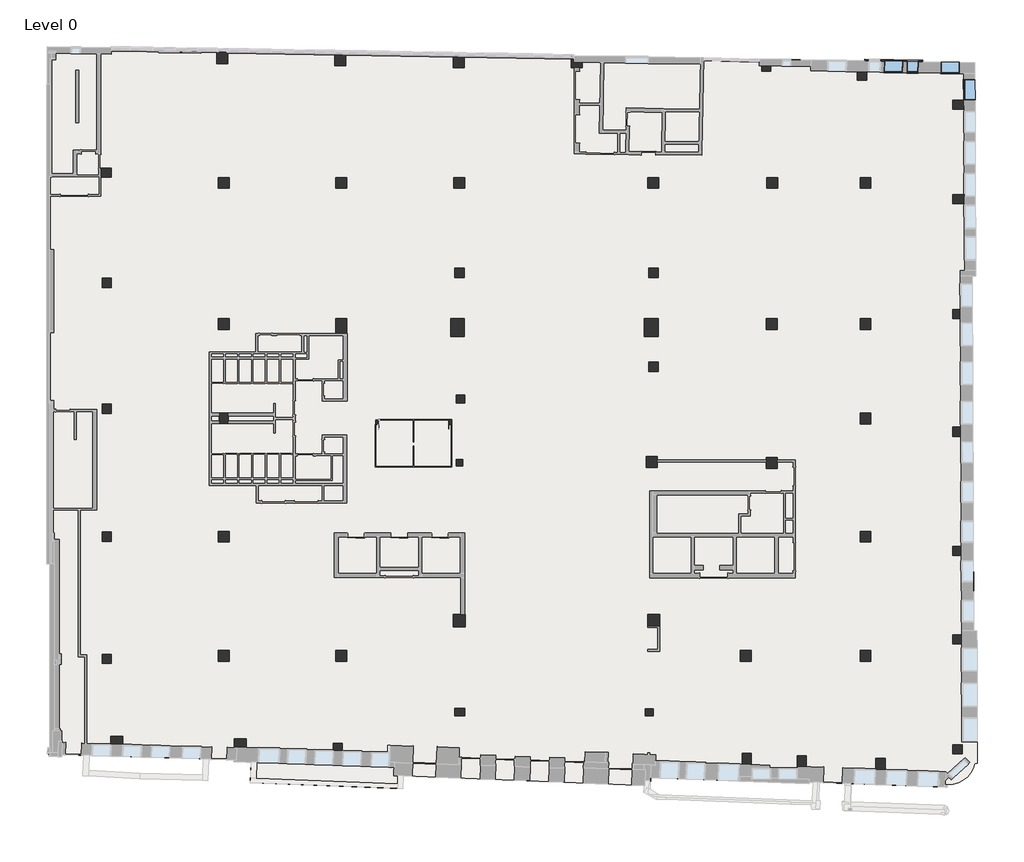
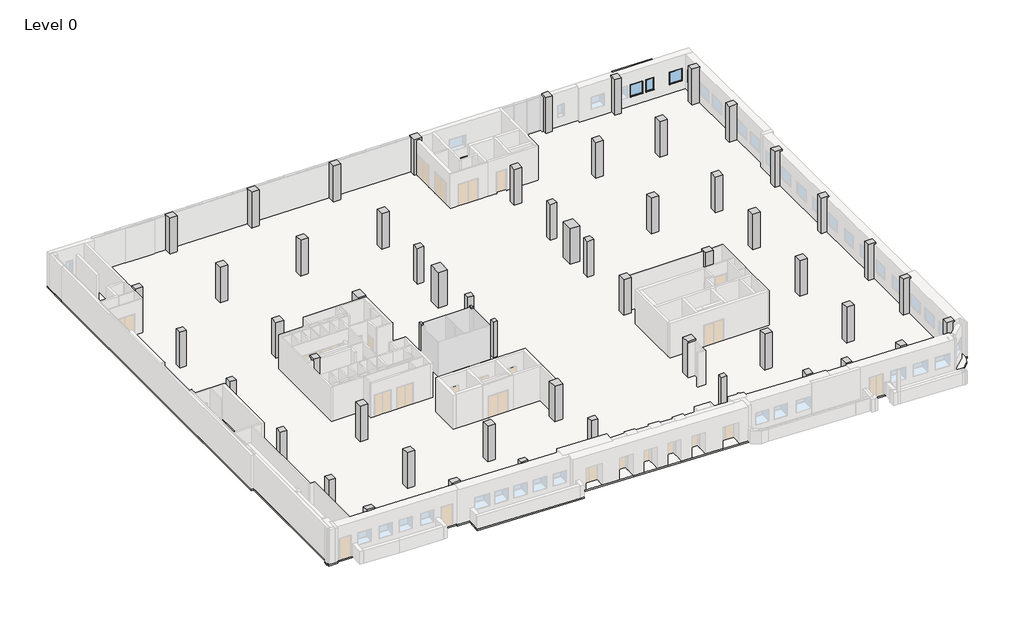
# One storey, part 9 of 9: 57 columns, 4 windows, 1 slab, 1 wall.
# Revit data of these elements (continued)
# Type "WWm-ConcreteRectangular-Instance : Generic" (continued)
#   Material = WW-EC-CR-CastInPlace
#   Assembly Code = ""
# Type "WWm-Existing-Slab-150mm"
#   Layers, outside or top first: 150 mm "WW-EC-CR-CastInPlace" (function 1)
# Type "WWm-Existing-ExtPartition-110mm"
#   Keynote = ""
#   Type IfcGUID = ""
#   Type Comments = ""
#   Description = ""
#   Type Mark = ""
#   Fire Rating = ""
#   Layers, outside or top first: 110 mm "WW-EC-RGB-White" (function 1)
# Type "Window-Instance : 1200x1200"
#   Type Mark = "11"
#   Construction Type Id = "GSP4R"
#   Assembly Code = "B2020100"
#   Analytic Construction = "1/8 in Pilkington single glazing"
#   Visual Light Transmittance = 0.9
#   Thermal Resistance (R) = 0.149095 (m²·K)/W
#   Solar Heat Gain Coefficient = 0.86
#   Heat Transfer Coefficient (U) = 6.70716 W/(m²·K)
#   Height [instance default] = 1200 mm
#   Default Sill Height = 900 mm
#   Width [instance default] = 600 mm
#   Window Inset = 20 mm
#   Glass Pane Material = none
#   Sash Material = none
#   Wall Closure = (empty or 0)
# Type "Window-Instance : 600x1200"
#   Type Mark = "7"
#   Construction Type Id = "GSP4R"
#   Assembly Code = "B2020100"
#   Analytic Construction = "1/8 in Pilkington single glazing"
#   Visual Light Transmittance = 0.9
#   Thermal Resistance (R) = 0.149095 (m²·K)/W
#   Solar Heat Gain Coefficient = 0.86
#   Heat Transfer Coefficient (U) = 6.70716 W/(m²·K)
#   Height [instance default] = 1200 mm
#   Default Sill Height = 900 mm
#   Width [instance default] = 600 mm
#   Window Inset = 20 mm
#   Glass Pane Material = WW-EC-GL-Storefront
#   Sash Material = WW-EC-RGB-White
#   Wall Closure = (empty or 0)
# Element 1 (IfcColumn, "WWm-ConcreteRectangular-Instance : Generic")
#   Width = 696 mm
#   Depth = 714.449 mm
#   Phase Created = Existing
#   Materials on its faces: "WW-EC-CR-CastInPlace", "WW-EC-RGB-White"
# Elements 2, 3, 4 (IfcColumn, "WWm-ConcreteRectangular-Instance : Generic")
#   Width = 696 mm
#   Depth = 692 mm
#   Phase Created = Existing
#   Materials on its faces: "WW-EC-CR-CastInPlace", "WW-EC-RGB-White"
# Elements 5, 6, 12, 19, 20, 21, 22, 23, 25, 26, 27, 29, 30, 31, 32, 33, 40, 57 (IfcColumn, "WWm-ConcreteRectangular-Instance : Generic")
#   Width = 696 mm
#   Depth = 692 mm
#   Phase Created = Existing
#   Materials on its faces: "WW-EC-CR-CastInPlace"
# Elements 7, 50, 51, 52 (IfcColumn, "WWm-ConcreteRectangular-Instance : Generic")
#   Width = 696 mm
#   Depth = 592 mm
#   Phase Created = Existing
#   Materials on its faces: "WW-EC-CR-CastInPlace", "WW-EC-RGB-White"
# Elements 8, 9, 11, 13, 34, 35 (IfcColumn, "WWm-ConcreteRectangular-Instance : Generic")
#   Width = 592 mm
#   Depth = 592 mm
#   Phase Created = Existing
#   Materials on its faces: "WW-EC-CR-CastInPlace"
# Element 10 (IfcColumn, "WWm-ConcreteRectangular-Instance : Generic")
#   Width = 600 mm
#   Depth = 669 mm
#   Phase Created = Existing
#   Materials on its faces: "WW-EC-CR-CastInPlace"
# Element 14 (IfcColumn, "WWm-ConcreteRectangular-Instance : Generic")
#   Width = 750 mm
#   Depth = 521.22 mm
#   Phase Created = Existing
#   Materials on its faces: "WW-EC-CR-CastInPlace", "WW-EC-RGB-White"
# Element 15 (IfcColumn, "WWm-ConcreteRectangular-Instance : Generic")
#   Width = 750 mm
#   Depth = 548.855 mm
#   Phase Created = Existing
#   Materials on its faces: "WW-EC-CR-CastInPlace", "WW-EC-RGB-White"
# Element 16 (IfcColumn, "WWm-ConcreteRectangular-Instance : Generic")
#   Width = 589.75 mm
#   Depth = 455.168 mm
#   Phase Created = Existing
#   Materials on its faces: "WW-EC-CR-CastInPlace", "WW-EC-RGB-White"
# Element 17 (IfcColumn, "WWm-ConcreteRectangular-Instance : Generic")
#   Width = 625.153 mm
#   Depth = 492.025 mm
#   Phase Created = Existing
#   Materials on its faces: "WW-EC-CR-CastInPlace"
# Element 18 (IfcColumn, "WWm-ConcreteRectangular-Instance : Generic")
#   Width = 498.218 mm
#   Depth = 470.145 mm
#   Phase Created = Existing
#   Materials on its faces: "WW-EC-CR-CastInPlace"
# Element 24 (IfcColumn, "WWm-ConcreteRectangular-Instance : Generic")
#   Width = 751 mm
#   Depth = 816 mm
#   Phase Created = Existing
#   Materials on its faces: "WW-EC-CR-CastInPlace"
# Element 28 (IfcColumn, "WWm-ConcreteRectangular-Instance : Generic")
#   Width = 696 mm
#   Depth = 966 mm
#   Phase Created = Existing
#   Materials on its faces: "WW-EC-CR-CastInPlace"
# Elements 36, 37 (IfcColumn, "WWm-ConcreteRectangular-Instance : Generic")
#   Width = 592 mm
#   Depth = 692 mm
#   Phase Created = Existing
#   Materials on its faces: "WW-EC-CR-CastInPlace", "WW-EC-RGB-White"
# Element 38 (IfcColumn, "WWm-ConcreteRectangular-Instance : Generic")
#   Width = 840.752 mm
#   Depth = 1139 mm
#   Phase Created = Existing
#   Materials on its faces: "WW-EC-CR-CastInPlace"
# Element 39 (IfcColumn, "WWm-ConcreteRectangular-Instance : Generic")
#   Width = 531.215 mm
#   Depth = 499.384 mm
#   Phase Created = Existing
#   Materials on its faces: "WW-EC-CR-CastInPlace"
# Element 41 (IfcColumn, "WWm-ConcreteRectangular-Instance : Generic")
#   Width = 592 mm
#   Depth = 627.436 mm
#   Phase Created = Existing
#   Materials on its faces: "WW-EC-CR-CastInPlace"
# Element 42 (IfcColumn, "WWm-ConcreteRectangular-Instance : Generic")
#   Width = 751.5 mm
#   Depth = 741 mm
#   Phase Created = Existing
#   Materials on its faces: "WW-EC-CR-CastInPlace"
# Element 43 (IfcColumn, "WWm-ConcreteRectangular-Instance : Generic")
#   Width = 886.756 mm
#   Depth = 1139 mm
#   Phase Created = Existing
#   Materials on its faces: "WW-EC-CR-CastInPlace"
# Element 44 (IfcColumn, "WWm-ConcreteRectangular-Instance : Generic")
#   Width = 169.771 mm
#   Depth = 284.187 mm
#   Phase Created = Existing
#   Materials on its faces: "WW-EC-CR-CastInPlace"
# Element 45 (IfcColumn, "WWm-ConcreteRectangular-Instance : Generic")
#   Width = 296.187 mm
#   Depth = 179.25 mm
#   Phase Created = Existing
#   Materials on its faces: "WW-EC-CR-CastInPlace"
# Element 46 (IfcColumn, "WWm-ConcreteRectangular-Instance : Generic")
#   Width = 573.511 mm
#   Depth = 685.737 mm
#   Phase Created = Existing
#   Materials on its faces: "WW-EC-CR-CastInPlace", "WW-EC-RGB-White"
# Element 47 (IfcColumn, "WWm-ConcreteRectangular-Instance : Generic")
#   Width = 571 mm
#   Depth = 692 mm
#   Phase Created = Existing
#   Materials on its faces: "WW-EC-CR-CastInPlace", "WW-EC-RGB-White"
# Element 48 (IfcColumn, "WWm-ConcreteRectangular-Instance : Generic")
#   Width = 600 mm
#   Depth = 712.368 mm
#   Phase Created = Existing
#   Materials on its faces: "WW-EC-CR-CastInPlace", "WW-EC-RGB-White"
# Element 49 (IfcColumn, "WWm-ConcreteRectangular-Instance : Generic")
#   Width = 696 mm
#   Depth = 550 mm
#   Phase Created = Existing
#   Materials on its faces: "WW-EC-CR-CastInPlace", "WW-EC-RGB-White"
# Elements 53, 54 (IfcColumn, "WWm-ConcreteRectangular-Instance : Generic")
#   Width = 734.7 mm
#   Depth = 585.57 mm
#   Phase Created = Existing
#   Materials on its faces: "WW-EC-CR-CastInPlace", "WW-EC-RGB-White"
# Element 55 (IfcColumn, "WWm-ConcreteRectangular-Instance : Generic")
#   Width = 696 mm
#   Depth = 571.35 mm
#   Phase Created = Existing
#   Materials on its faces: "WW-EC-CR-CastInPlace", "WW-EC-RGB-White"
# Element 56 (IfcColumn, "WWm-ConcreteRectangular-Instance : Generic")
#   Width = 400 mm
#   Depth = 400 mm
#   Phase Created = Existing
#   Materials on its faces: "WW-EC-CR-CastInPlace"
# Element 58 (IfcSlab, "WWm-Existing-Slab-150mm")
#   built-in parameter 1001955 = 3.12418 (stored number, unit not read)
#   Height Offset From Level = 0 mm
#   Phase Created = Existing
#   Materials on its faces: "WW-EC-CR-CastInPlace"
# Element 59 (IfcWall, "WWm-Existing-ExtPartition-110mm")
#   Top Offset = -150 mm
#   Base Offset = 0 mm
#   wall height = 3350 mm
#   Phase Created = Existing
#   Base Constraint = Level 0
#   Top Constraint = Level 1
#   Materials on its faces: "WW-EC-RGB-White"
# Element 60 (IfcWindow, "Window-Instance : 1200x1200")
#   Mark = "12"
#   Width = 1200 mm
#   Height = 1200 mm
#   Phase Created = Existing
# Element 61 (IfcWindow, "Window-Instance : 600x1200")
#   Mark = "13"
#   Width = 750 mm
#   Height = 1200 mm
#   Phase Created = Existing
#   Materials on its faces: "WW-EC-RGB-White", "WW-EC-GL-Storefront"
# Element 62 (IfcWindow, "Window-Instance : 600x1200")
#   Mark = "14"
#   Width = 1200 mm
#   Height = 1200 mm
#   Phase Created = Existing
#   Materials on its faces: "WW-EC-RGB-White", "WW-EC-GL-Storefront"
# Element 63 (IfcWindow, "Window-Instance : 600x1200")
#   Mark = "15"
#   Width = 1350 mm
#   Height = 1200 mm
#   Phase Created = Existing
#   Materials on its faces: "WW-EC-RGB-White", "WW-EC-GL-Storefront"
# Materials
#   "WW-EC-CR-CastInPlace": class "Concrete", colour RGB 255 255 255, transparency 0, Comments = "If region requests all-white model, remove image from asset", Description = "Cast in Place Concrete", Cost = 0
#   "WW-EC-RGB-White": class "Generic", colour RGB 255 255 255, transparency 0, Comments = "If region requests off-white, swith asset color to RGB 231-228-220", Description = "Generic Color", Cost = 0
#   "WW-EC-GL-Storefront": class "Glass", colour RGB 236 240 239, transparency 0.85, Description = "Storefront Glass", Cost = 0
